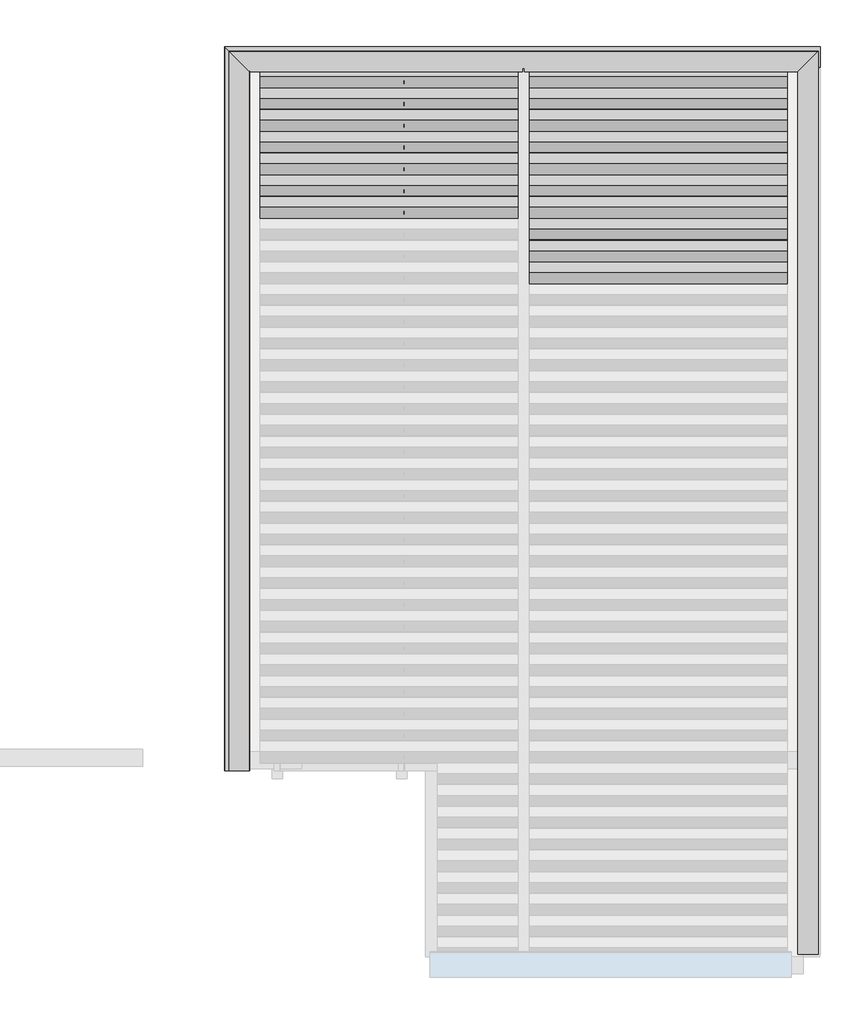
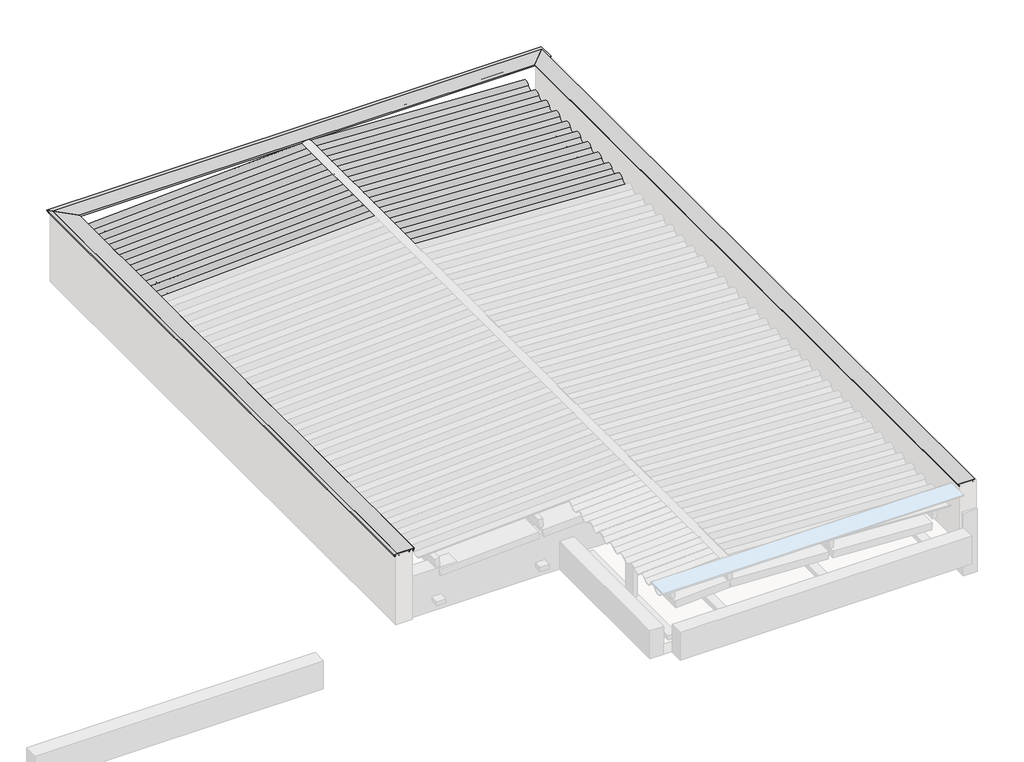
# One storey, part 4 of 4: 23 beams, 5 columns, 3 proxies.
"""IFC4 building model written with IfcOpenShell, lengths in millimetres."""

import ifcopenshell
import ifcopenshell.guid

model = None  # the IFC model being written
_history = None  # IfcOwnerHistory: only IFC2X3 demands one
_inside = {}  # id of a spatial element -> (the spatial element, [elements in it])
_under = {}  # id of a project, library or spatial element -> (it, [spatial elements below it])
_declared = {}  # id of a project -> (the project, [libraries it declares])
_typed = {}  # id of a type object -> (the type object, [elements of that type])
_made_of = {}  # id of a material, layer set ... -> (it, [elements and type objects made of it])


def new_model(schema):
    """Start an empty IFC model of exactly this schema.

    Asked for "IFC4X3", IfcOpenShell would pick the latest addendum, in which some entities
    have other attributes; the version numbers below select the first issue.
    IFC2X3 requires an IfcOwnerHistory on every rooted entity: one is made here for all.
    """
    global model, _history
    if schema == "IFC4X3":
        model = ifcopenshell.file(schema_version=(4, 3, 0, 0))
    else:
        model = ifcopenshell.file(schema=schema)
    _inside.clear()
    _under.clear()
    _declared.clear()
    _typed.clear()
    _made_of.clear()
    _history = None
    if model.schema == "IFC2X3":
        org = make("IfcOrganization", Name="unknown")
        user = make(
            "IfcPersonAndOrganization",
            ThePerson=make("IfcPerson", FamilyName="unknown"),
            TheOrganization=org,
        )
        app = make(
            "IfcApplication",
            ApplicationDeveloper=org,
            Version="unknown",
            ApplicationFullName="unknown",
            ApplicationIdentifier="unknown",
        )
        _history = make(
            "IfcOwnerHistory",
            OwningUser=user,
            OwningApplication=app,
            ChangeAction="ADDED",
            CreationDate=0,
        )
    return model


def make(cls, **values):
    """One entity of the class cls with the attributes given. An attribute that is None is left unset."""
    return model.create_entity(
        cls, **{name: value for name, value in values.items() if value is not None}
    )


def rooted(cls, **values):
    """An entity with a GlobalId (a new one), such as an element, a storey or a relation."""
    return make(cls, GlobalId=ifcopenshell.guid.new(), OwnerHistory=_history, **values)


def si_unit(unit_type, name, prefix=None):
    """IfcSIUnit, for example si_unit("LENGTHUNIT", "METRE", prefix="MILLI")."""
    return make("IfcSIUnit", UnitType=unit_type, Prefix=prefix, Name=name)


def assignment(units):
    """IfcUnitAssignment: the units of a project."""
    return None if units is None else make("IfcUnitAssignment", Units=units)


def point(xyz):
    """IfcCartesianPoint."""
    return None if xyz is None else make("IfcCartesianPoint", Coordinates=xyz)


def direction(xyz):
    """IfcDirection."""
    return None if xyz is None else make("IfcDirection", DirectionRatios=xyz)


def frame(location, z_axis=None, x_axis=None):
    """IfcAxis2Placement3D, a coordinate frame: its origin and axes. An axis left out is left unset."""
    return make(
        "IfcAxis2Placement3D",
        Location=point(location),
        Axis=direction(z_axis),
        RefDirection=direction(x_axis),
    )


def frame_2d(location, x_axis=None):
    """IfcAxis2Placement2D, a coordinate frame in the plane: its origin and x axis."""
    return make(
        "IfcAxis2Placement2D", Location=point(location), RefDirection=direction(x_axis)
    )


def origin():
    """The frame at (0, 0, 0) with its axes left unset."""
    return frame((0.0, 0.0, 0.0))


def place(relative_to, where):
    """IfcLocalPlacement: puts the frame where relative to a parent placement (None: the world)."""
    return make(
        "IfcLocalPlacement", PlacementRelTo=relative_to, RelativePlacement=where
    )


def context(
    kind, dimensions, precision=None, world=None, true_north=None, identifier=None
):
    """IfcGeometricRepresentationContext, for example the 3D "Model" context."""
    return make(
        "IfcGeometricRepresentationContext",
        ContextIdentifier=identifier,
        ContextType=kind,
        CoordinateSpaceDimension=dimensions,
        Precision=precision,
        WorldCoordinateSystem=world,
        TrueNorth=true_north,
    )


def project(units=None, contexts=None):
    """IfcProject with its units and contexts."""
    return rooted(
        "IfcProject",
        Name="project",
        RepresentationContexts=contexts,
        UnitsInContext=assignment(units),
    )


def spatial(cls, under=None, at=None, **own):
    """A site, building, storey or space (cls), placed at a placement, below another one or the project."""
    s = rooted(cls, ObjectPlacement=at, **own)
    if under is not None:
        _under.setdefault(under.id(), (under, []))[1].append(s)
    return s


def polyline(points):
    """IfcPolyline through the points."""
    return make("IfcPolyline", Points=[point(p) for p in points])


def circle_curve(where, radius):
    """IfcCircle in the frame where."""
    return make("IfcCircle", Position=where, Radius=radius)


def trimmed(basis, trim1, trim2, sense, master):
    """IfcTrimmedCurve: the piece of a basis curve between two trims."""
    return make(
        "IfcTrimmedCurve",
        BasisCurve=basis,
        Trim1=trim1,
        Trim2=trim2,
        SenseAgreement=sense,
        MasterRepresentation=master,
    )


def segment(curve, same_sense, transition):
    """IfcCompositeCurveSegment."""
    return make(
        "IfcCompositeCurveSegment",
        Transition=transition,
        SameSense=same_sense,
        ParentCurve=curve,
    )


def composite_curve(segments, self_intersect=None):
    """IfcCompositeCurve: segments joined end to end."""
    return make("IfcCompositeCurve", Segments=segments, SelfIntersect=self_intersect)


def outline(outer, holes=None, kind="AREA"):
    """IfcArbitraryClosedProfileDef: a profile drawn as a closed curve; with holes, ...WithVoids."""
    if holes is None:
        return make("IfcArbitraryClosedProfileDef", ProfileType=kind, OuterCurve=outer)
    return make(
        "IfcArbitraryProfileDefWithVoids",
        ProfileType=kind,
        OuterCurve=outer,
        InnerCurves=holes,
    )


def extrude(swept, where, along, depth):
    """IfcExtrudedAreaSolid: the profile swept, set in the frame where, extruded along a direction by depth."""
    return make(
        "IfcExtrudedAreaSolid",
        SweptArea=swept,
        Position=where,
        ExtrudedDirection=direction(along),
        Depth=depth,
    )


def faces_of(points, faces, orient=None, outer=None):
    """IfcFace entities. A face is a list of loops; a loop is a list of indices into points, from 0.

    orient and outer hold one flag for each loop. By default every Orientation is true, the
    first loop of a face is its IfcFaceOuterBound and the others are IfcFaceBound.
    """
    made = []
    for i, loops in enumerate(faces):
        bounds = []
        for j, loop in enumerate(loops):
            is_outer = j == 0 if outer is None else outer[i][j]
            bounds.append(
                make(
                    "IfcFaceOuterBound" if is_outer else "IfcFaceBound",
                    Bound=make("IfcPolyLoop", Polygon=[points[k] for k in loop]),
                    Orientation=True if orient is None else orient[i][j],
                )
            )
        made.append(make("IfcFace", Bounds=bounds))
    return made


def faceted_brep(points, faces, orient=None, outer=None, voids=None):
    """IfcFacetedBrep: a solid bounded by flat faces; with voids (closed shells), ...WithVoids."""
    shared = [point(p) for p in points]
    hull = make("IfcClosedShell", CfsFaces=faces_of(shared, faces, orient, outer))
    if voids is None:
        return make("IfcFacetedBrep", Outer=hull)
    return make(
        "IfcFacetedBrepWithVoids",
        Outer=hull,
        Voids=[
            make(cls, CfsFaces=faces_of(shared, fs, o, b)) for cls, fs, o, b in voids
        ],
    )


def shape(context_of_items, identifier, shape_type, items):
    """IfcShapeRepresentation: the items that make up one representation, for example the "Body"."""
    return make(
        "IfcShapeRepresentation",
        ContextOfItems=context_of_items,
        RepresentationIdentifier=identifier,
        RepresentationType=shape_type,
        Items=items,
    )


def source(mapping_origin, context_of_items, identifier, shape_type, items):
    """IfcRepresentationMap: a shape defined once, which mapped items show again and again."""
    return make(
        "IfcRepresentationMap",
        MappingOrigin=mapping_origin,
        MappedRepresentation=shape(context_of_items, identifier, shape_type, items),
    )


def transform(
    local_origin,
    x_axis=None,
    y_axis=None,
    z_axis=None,
    scale=None,
    scale2=None,
    scale3=None,
    uniform=True,
):
    """IfcCartesianTransformationOperator3D, or its non-uniform kind. x_axis, y_axis, z_axis: its Axis1, 2, 3."""
    if uniform:
        return make(
            "IfcCartesianTransformationOperator3D",
            Axis1=direction(x_axis),
            Axis2=direction(y_axis),
            LocalOrigin=point(local_origin),
            Scale=scale,
            Axis3=direction(z_axis),
        )
    return make(
        "IfcCartesianTransformationOperator3DnonUniform",
        Axis1=direction(x_axis),
        Axis2=direction(y_axis),
        LocalOrigin=point(local_origin),
        Scale=scale,
        Axis3=direction(z_axis),
        Scale2=scale2,
        Scale3=scale3,
    )


def mapped(mapping_source, mapping_target):
    """IfcMappedItem: shows the shape of a source again, moved by a transform."""
    return make(
        "IfcMappedItem", MappingSource=mapping_source, MappingTarget=mapping_target
    )


def made_of(thing, what):
    """Note that an element or type object is made of a material, layer set ...; save() writes the relation."""
    if what is not None:
        _made_of.setdefault(what.id(), (what, []))[1].append(thing)
    return thing


def element(
    cls,
    number,
    at=None,
    inside=None,
    cuts=None,
    type_object=None,
    material=None,
    context=None,
    identifier="Body",
    shape_type=None,
    held_by="IfcProductDefinitionShape",
    body=None,
    shapes=None,
    **own,
):
    """One element of the class cls, such as IfcWall. Its Tag is "e" and its number.

    at: its placement. inside: the storey or other place that contains it. cuts: it is an
    opening in that element (IfcRelVoidsElement). A single representation is given by context,
    identifier, shape_type and body (its items); several are given by shapes. held_by: the class
    of the entity that holds the representations. save() writes the other relations.
    """
    e = rooted(cls, Tag="e%d" % number, ObjectPlacement=at, **own)
    if body is not None:
        shapes = [shape(context, identifier, shape_type, body)]
    if shapes is not None:
        e.Representation = make(held_by, Representations=shapes)
    if inside is not None:
        _inside.setdefault(inside.id(), (inside, []))[1].append(e)
    if cuts is not None:
        rooted(
            "IfcRelVoidsElement", RelatingBuildingElement=cuts, RelatedOpeningElement=e
        )
    if type_object is not None:
        _typed.setdefault(type_object.id(), (type_object, []))[1].append(e)
    return made_of(e, material)


def aggregate(whole, parts):
    """IfcRelAggregates: a whole, such as a stair, and the parts it consists of."""
    return rooted("IfcRelAggregates", RelatingObject=whole, RelatedObjects=parts)


def save(model, path):
    """Write the relations noted so far, then the file.

    IfcRelAggregates (storeys below a building ...), IfcRelContainedInSpatialStructure (elements
    in a storey), IfcRelDefinesByType, IfcRelAssociatesMaterial and IfcRelDeclares: one each for
    every whole, place, type object, material and project.
    """
    for whole, parts in _under.values():
        aggregate(whole, parts)
    for where, things in _inside.values():
        rooted(
            "IfcRelContainedInSpatialStructure",
            RelatedElements=things,
            RelatingStructure=where,
        )
    for kind, things in _typed.values():
        rooted("IfcRelDefinesByType", RelatedObjects=things, RelatingType=kind)
    for what, things in _made_of.values():
        rooted("IfcRelAssociatesMaterial", RelatedObjects=things, RelatingMaterial=what)
    for by, libraries in _declared.values():
        rooted("IfcRelDeclares", RelatingContext=by, RelatedDefinitions=libraries)
    model.write(path)


def column_f3930958(model_context):
    return source(origin(), model_context, "Body", "SweptSolid", [
        extrude(outline(polyline([(30.0, 80.0), (30.0, -80.0), (-30.0, -80.0), (-30.0, 80.0), (30.0, 80.0)])), frame((0.0, 0.0, 4460.0), z_axis=(0.0, 0.0, 1.0), x_axis=(1.0, 0.0, 0.0)), (0.0, 0.0, 1.0), 522.9),
    ])


def column_4d3918cc(model_context):
    return source(origin(), model_context, "Body", "SweptSolid", [
        extrude(outline(polyline([(30.0, 80.0), (30.0, -80.0), (-30.0, -80.0), (-30.0, 80.0), (30.0, 80.0)])), frame((0.0, 0.0, 4460.0), z_axis=(0.0, 0.0, 1.0), x_axis=(1.0, 0.0, 0.0)), (0.0, 0.0, 1.0), 426.9),
    ])


def column_924cc83b(model_context):
    return source(origin(), model_context, "Body", "SweptSolid", [
        extrude(outline(polyline([(30.0, 80.0), (30.0, -80.0), (-30.0, -80.0), (-30.0, 80.0), (30.0, 80.0)])), frame((0.0, 0.0, 4460.0), z_axis=(0.0, 0.0, 1.0), x_axis=(1.0, 0.0, 0.0)), (0.0, 0.0, 1.0), 497.0),
    ])


model = new_model("IFC4")

# Units and contexts
model_context = context("Model", 3, world=origin())
ifc_project = project(units=[si_unit("LENGTHUNIT", "METRE", prefix="MILLI")], contexts=[model_context])

# Site, building, storey
site = spatial("IfcSite", under=ifc_project)
building = spatial("IfcBuilding", under=site)
storey = spatial("IfcBuildingStorey", under=building, Name="COB. SALA ESTAR", Elevation=4400.0)

# Beams
placement = place(None, origin())
element("IfcBeam", 1, ObjectType="Madeira de lei : Berço 6x12cm", at=placement, inside=storey, context=model_context, shape_type="SweptSolid", body=[
    extrude(outline(polyline([(-3400.781307, 5593.9300153), (-3280.781307, 5593.9300153), (-3280.781307, 3623.9300153), (-3400.781307, 3623.9300153), (-3400.781307, 5593.9300153)])), frame((0.0, 0.0, 4400.0), z_axis=(0.0, 0.0, 1.0), x_axis=(1.0, 0.0, 0.0)), (0.0, 0.0, 1.0), 60.0),
])
element("IfcBeam", 2, ObjectType="Madeira de lei : Berço 6x12cm", at=placement, inside=storey, context=model_context, shape_type="SweptSolid", body=[
    extrude(outline(polyline([(-2032.4438771, 5593.9300153), (-1912.4438771, 5593.9300153), (-1912.4438771, 3623.9300153), (-2032.4438771, 3623.9300153), (-2032.4438771, 5593.9300153)])), frame((0.0, 0.0, 4400.0), z_axis=(0.0, 0.0, 1.0), x_axis=(1.0, 0.0, 0.0)), (0.0, 0.0, 1.0), 60.0),
])
element("IfcBeam", 3, ObjectType="Madeira de lei : Berço 6x12cm", at=placement, inside=storey, context=model_context, shape_type="SweptSolid", body=[
    extrude(outline(polyline([(-634.1438771, 5593.9300153), (-514.1438771, 5593.9300153), (-514.1438771, 3623.9300153), (-634.1438771, 3623.9300153), (-634.1438771, 5593.9300153)])), frame((0.0, 0.0, 4400.0), z_axis=(0.0, 0.0, 1.0), x_axis=(1.0, 0.0, 0.0)), (0.0, 0.0, 1.0), 60.0),
])
element("IfcBeam", 4, ObjectType="Madeira de lei : Berço 6x12cm", at=placement, inside=storey, context=model_context, shape_type="SweptSolid", body=[
    extrude(outline(polyline([(-4769.1187368, 5593.9300153), (-4649.1187368, 5593.9300153), (-4649.1187368, 3623.9300153), (-4769.1187368, 3623.9300153), (-4769.1187368, 5593.9300153)])), frame((0.0, 0.0, 4400.0), z_axis=(0.0, 0.0, 1.0), x_axis=(1.0, 0.0, 0.0)), (0.0, 0.0, 1.0), 60.0),
])
element("IfcBeam", 5, ObjectType="Madeira de lei : Berço 6x12cm", at=placement, inside=storey, context=model_context, shape_type="SweptSolid", body=[
    extrude(outline(polyline([(-6167.4187368, 5593.9300153), (-6047.4187368, 5593.9300153), (-6047.4187368, 3623.9300153), (-6167.4187368, 3623.9300153), (-6167.4187368, 5593.9300153)])), frame((0.0, 0.0, 4400.0), z_axis=(0.0, 0.0, 1.0), x_axis=(1.0, 0.0, 0.0)), (0.0, 0.0, 1.0), 60.0),
])
element("IfcBeam", 6, ObjectType="TQS - Viga retangular : 19.0 x 60.0", at=placement, inside=storey, context=model_context, shape_type="SweptSolid", body=[
    extrude(outline(polyline([(-412.281307, 5774.4300153), (-412.281307, 5584.4300153), (-6230.281307, 5584.4300153), (-6230.281307, 5774.4300153), (-412.281307, 5774.4300153)])), frame((0.0, 0.0, 4250.0), z_axis=(0.0, 0.0, 1.0), x_axis=(1.0, 0.0, 0.0)), (0.0, 0.0, 1.0), 600.0),
])
element("IfcBeam", 7, ObjectType="Telha Ondulada : Fibrocimento", at=placement, inside=storey, context=model_context, shape_type="SweptSolid", body=[
    extrude(outline(composite_curve([segment(trimmed(circle_curve(frame_2d((-58.7002978, -53.2060538)), 66.7939461), [point((-29.3501488, 6.7939462))], [point((-29.3501488, -113.2060538))], False, "CARTESIAN"), True, "CONTINUOUS"), segment(polyline([(-29.3501488, -113.2060538), (-31.5472154, -108.7146288)]), True, "CONTINUOUS"), segment(trimmed(circle_curve(frame_2d((-58.7002978, -53.2060538)), 61.7939461), [point((-31.5472154, -108.7146288))], [point((-31.5472154, 2.3025211))], True, "CARTESIAN"), True, "CONTINUOUS"), segment(trimmed(circle_curve(frame_2d((0.0, 66.7939462)), 71.7939461), [point((-31.5472154, 2.3025211))], [point((-31.5472154, 131.2853712))], False, "CARTESIAN"), True, "CONTINUOUS"), segment(polyline([(-31.5472154, 131.2853712), (-29.3501488, 126.7939462)]), True, "CONTINUOUS"), segment(trimmed(circle_curve(frame_2d((0.0, 66.7939462)), 66.7939461), [point((-29.3501488, 126.7939462))], [point((-29.3501488, 6.7939462))], True, "CARTESIAN"), True, "CONTINUOUS")], self_intersect=False)), frame((-6303.6781287, 4045.326948, 5068.1236978), z_axis=(0.9987523388778448, 0.0, 0.04993761694389136), x_axis=(-0.04993761694389136, 0.0, 0.9987523388778448)), (0.0, 0.0, 1.0), 2962.0084336),
])
element("IfcBeam", 8, ObjectType="Telha Ondulada : Fibrocimento", at=placement, inside=storey, context=model_context, shape_type="SweptSolid", body=[
    extrude(outline(composite_curve([segment(trimmed(circle_curve(frame_2d((-58.7002978, -53.2060538)), 66.7939461), [point((-29.3501488, 6.7939462))], [point((-29.3501488, -113.2060538))], False, "CARTESIAN"), True, "CONTINUOUS"), segment(polyline([(-29.3501488, -113.2060538), (-31.5472154, -108.7146288)]), True, "CONTINUOUS"), segment(trimmed(circle_curve(frame_2d((-58.7002978, -53.2060538)), 61.7939461), [point((-31.5472154, -108.7146288))], [point((-31.5472154, 2.3025211))], True, "CARTESIAN"), True, "CONTINUOUS"), segment(trimmed(circle_curve(frame_2d((0.0, 66.7939462)), 71.7939461), [point((-31.5472154, 2.3025211))], [point((-31.5472154, 131.2853712))], False, "CARTESIAN"), True, "CONTINUOUS"), segment(polyline([(-31.5472154, 131.2853712), (-29.3501488, 126.7939462)]), True, "CONTINUOUS"), segment(trimmed(circle_curve(frame_2d((0.0, 66.7939462)), 66.7939461), [point((-29.3501488, 126.7939462))], [point((-29.3501488, 6.7939462))], True, "CARTESIAN"), True, "CONTINUOUS")], self_intersect=False)), frame((-6303.6781287, 4289.826948, 5068.1236978), z_axis=(0.9987523388778448, 0.0, 0.04993761694389134), x_axis=(-0.04993761694389134, 0.0, 0.9987523388778448)), (0.0, 0.0, 1.0), 2962.0084336),
])
element("IfcBeam", 9, ObjectType="Telha Ondulada : Fibrocimento", at=placement, inside=storey, context=model_context, shape_type="SweptSolid", body=[
    extrude(outline(composite_curve([segment(trimmed(circle_curve(frame_2d((-58.7002978, -53.2060538)), 66.7939461), [point((-29.3501488, 6.7939462))], [point((-29.3501488, -113.2060538))], False, "CARTESIAN"), True, "CONTINUOUS"), segment(polyline([(-29.3501488, -113.2060538), (-31.5472154, -108.7146288)]), True, "CONTINUOUS"), segment(trimmed(circle_curve(frame_2d((-58.7002978, -53.2060538)), 61.7939461), [point((-31.5472154, -108.7146288))], [point((-31.5472154, 2.3025211))], True, "CARTESIAN"), True, "CONTINUOUS"), segment(trimmed(circle_curve(frame_2d((0.0, 66.7939462)), 71.7939461), [point((-31.5472154, 2.3025211))], [point((-31.5472154, 131.2853712))], False, "CARTESIAN"), True, "CONTINUOUS"), segment(polyline([(-31.5472154, 131.2853712), (-29.3501488, 126.7939462)]), True, "CONTINUOUS"), segment(trimmed(circle_curve(frame_2d((0.0, 66.7939462)), 66.7939461), [point((-29.3501488, 126.7939462))], [point((-29.3501488, 6.7939462))], True, "CARTESIAN"), True, "CONTINUOUS")], self_intersect=False)), frame((-6303.6781287, 4534.326948, 5068.1236978), z_axis=(0.9987523388778448, 0.0, 0.04993761694389133), x_axis=(-0.04993761694389133, 0.0, 0.9987523388778448)), (0.0, 0.0, 1.0), 2962.0084336),
])
element("IfcBeam", 10, ObjectType="Telha Ondulada : Fibrocimento", at=placement, inside=storey, context=model_context, shape_type="SweptSolid", body=[
    extrude(outline(composite_curve([segment(trimmed(circle_curve(frame_2d((-58.7002978, -53.2060538)), 66.7939461), [point((-29.3501488, 6.7939462))], [point((-29.3501488, -113.2060538))], False, "CARTESIAN"), True, "CONTINUOUS"), segment(polyline([(-29.3501488, -113.2060538), (-31.5472154, -108.7146288)]), True, "CONTINUOUS"), segment(trimmed(circle_curve(frame_2d((-58.7002978, -53.2060538)), 61.7939461), [point((-31.5472154, -108.7146288))], [point((-31.5472154, 2.3025211))], True, "CARTESIAN"), True, "CONTINUOUS"), segment(trimmed(circle_curve(frame_2d((0.0, 66.7939462)), 71.7939461), [point((-31.5472154, 2.3025211))], [point((-31.5472154, 131.2853712))], False, "CARTESIAN"), True, "CONTINUOUS"), segment(polyline([(-31.5472154, 131.2853712), (-29.3501488, 126.7939462)]), True, "CONTINUOUS"), segment(trimmed(circle_curve(frame_2d((0.0, 66.7939462)), 66.7939461), [point((-29.3501488, 126.7939462))], [point((-29.3501488, 6.7939462))], True, "CARTESIAN"), True, "CONTINUOUS")], self_intersect=False)), frame((-6303.6781287, 4778.826948, 5068.1236978), z_axis=(0.9987523388778448, 0.0, 0.049937616943891344), x_axis=(-0.049937616943891344, 0.0, 0.9987523388778448)), (0.0, 0.0, 1.0), 2962.0084336),
])
element("IfcBeam", 11, ObjectType="Telha Ondulada : Fibrocimento", at=placement, inside=storey, context=model_context, shape_type="SweptSolid", body=[
    extrude(outline(composite_curve([segment(trimmed(circle_curve(frame_2d((-58.7002978, -53.2060538)), 66.7939461), [point((-29.3501488, 6.7939462))], [point((-29.3501488, -113.2060538))], False, "CARTESIAN"), True, "CONTINUOUS"), segment(polyline([(-29.3501488, -113.2060538), (-31.5472154, -108.7146288)]), True, "CONTINUOUS"), segment(trimmed(circle_curve(frame_2d((-58.7002978, -53.2060538)), 61.7939461), [point((-31.5472154, -108.7146288))], [point((-31.5472154, 2.3025211))], True, "CARTESIAN"), True, "CONTINUOUS"), segment(trimmed(circle_curve(frame_2d((0.0, 66.7939462)), 71.7939461), [point((-31.5472154, 2.3025211))], [point((-31.5472154, 131.2853712))], False, "CARTESIAN"), True, "CONTINUOUS"), segment(polyline([(-31.5472154, 131.2853712), (-29.3501488, 126.7939462)]), True, "CONTINUOUS"), segment(trimmed(circle_curve(frame_2d((0.0, 66.7939462)), 66.7939461), [point((-29.3501488, 126.7939462))], [point((-29.3501488, 6.7939462))], True, "CARTESIAN"), True, "CONTINUOUS")], self_intersect=False)), frame((-6303.6781287, 5023.326948, 5068.1236978), z_axis=(0.9987523388778448, 0.0, 0.04993761694389134), x_axis=(-0.04993761694389134, 0.0, 0.9987523388778448)), (0.0, 0.0, 1.0), 2962.0084336),
])
element("IfcBeam", 12, ObjectType="Telha Ondulada : Fibrocimento", at=placement, inside=storey, context=model_context, shape_type="SweptSolid", body=[
    extrude(outline(composite_curve([segment(trimmed(circle_curve(frame_2d((-58.7002978, -53.2060538)), 66.7939461), [point((-29.3501488, 6.7939462))], [point((-29.3501488, -113.2060538))], False, "CARTESIAN"), True, "CONTINUOUS"), segment(polyline([(-29.3501488, -113.2060538), (-31.5472154, -108.7146288)]), True, "CONTINUOUS"), segment(trimmed(circle_curve(frame_2d((-58.7002978, -53.2060538)), 61.7939461), [point((-31.5472154, -108.7146288))], [point((-31.5472154, 2.3025211))], True, "CARTESIAN"), True, "CONTINUOUS"), segment(trimmed(circle_curve(frame_2d((0.0, 66.7939462)), 71.7939461), [point((-31.5472154, 2.3025211))], [point((-31.5472154, 131.2853712))], False, "CARTESIAN"), True, "CONTINUOUS"), segment(polyline([(-31.5472154, 131.2853712), (-29.3501488, 126.7939462)]), True, "CONTINUOUS"), segment(trimmed(circle_curve(frame_2d((0.0, 66.7939462)), 66.7939461), [point((-29.3501488, 126.7939462))], [point((-29.3501488, 6.7939462))], True, "CARTESIAN"), True, "CONTINUOUS")], self_intersect=False)), frame((-6303.6781287, 5267.826948, 5068.1236978), z_axis=(0.9987523388778448, 0.0, 0.04993761694389136), x_axis=(-0.04993761694389136, 0.0, 0.9987523388778448)), (0.0, 0.0, 1.0), 2962.0084336),
])
element("IfcBeam", 13, ObjectType="Telha Ondulada : Fibrocimento", at=placement, inside=storey, context=model_context, shape_type="SweptSolid", body=[
    extrude(outline(composite_curve([segment(trimmed(circle_curve(frame_2d((-58.7002978, -53.2060538)), 66.7939461), [point((-29.3501488, 6.7939462))], [point((-29.3501488, -113.2060538))], False, "CARTESIAN"), True, "CONTINUOUS"), segment(polyline([(-29.3501488, -113.2060538), (-31.5472154, -108.7146288)]), True, "CONTINUOUS"), segment(trimmed(circle_curve(frame_2d((-58.7002978, -53.2060538)), 61.7939461), [point((-31.5472154, -108.7146288))], [point((-31.5472154, 2.3025211))], True, "CARTESIAN"), True, "CONTINUOUS"), segment(trimmed(circle_curve(frame_2d((0.0, 66.7939462)), 71.7939461), [point((-31.5472154, 2.3025211))], [point((-31.5472154, 131.2853712))], False, "CARTESIAN"), True, "CONTINUOUS"), segment(polyline([(-31.5472154, 131.2853712), (-29.3501488, 126.7939462)]), True, "CONTINUOUS"), segment(trimmed(circle_curve(frame_2d((0.0, 66.7939462)), 66.7939461), [point((-29.3501488, 126.7939462))], [point((-29.3501488, 6.7939462))], True, "CARTESIAN"), True, "CONTINUOUS")], self_intersect=False)), frame((-6303.6781287, 5512.326948, 5068.1236978), z_axis=(0.9987523388778448, 0.0, 0.04993761694389134), x_axis=(-0.04993761694389134, 0.0, 0.9987523388778448)), (0.0, 0.0, 1.0), 2962.0084336),
])
element("IfcBeam", 14, ObjectType="Telha Ondulada : Fibrocimento", at=placement, inside=storey, context=model_context, shape_type="SweptSolid", body=[
    extrude(outline(composite_curve([segment(trimmed(circle_curve(frame_2d((0.0, 66.7939462)), 66.7939461), [point((29.3501488, 6.7939462))], [point((29.3501488, 126.7939462))], True, "CARTESIAN"), True, "CONTINUOUS"), segment(polyline([(29.3501488, 126.7939462), (31.5472154, 131.2853712)]), True, "CONTINUOUS"), segment(trimmed(circle_curve(frame_2d((0.0, 66.7939462)), 71.7939461), [point((31.5472154, 131.2853712))], [point((31.5472154, 2.3025211))], False, "CARTESIAN"), True, "CONTINUOUS"), segment(trimmed(circle_curve(frame_2d((58.7002978, -53.2060538)), 61.7939461), [point((31.5472154, 2.3025211))], [point((31.5472154, -108.7146288))], True, "CARTESIAN"), True, "CONTINUOUS"), segment(polyline([(31.5472154, -108.7146288), (29.3501488, -113.2060538)]), True, "CONTINUOUS"), segment(trimmed(circle_curve(frame_2d((58.7002978, -53.2060538)), 66.7939461), [point((29.3501488, -113.2060538))], [point((29.3501488, 6.7939462))], False, "CARTESIAN"), True, "CONTINUOUS")], self_intersect=False)), frame((-377.8844852, 3311.826948, 5068.1236978), z_axis=(-0.9987523388778448, 0.0, 0.049937616943891455), x_axis=(-0.049937616943891455, 0.0, -0.9987523388778448)), (0.0, 0.0, 1.0), 2962.0084336),
])
element("IfcBeam", 15, ObjectType="Telha Ondulada : Fibrocimento", at=placement, inside=storey, context=model_context, shape_type="SweptSolid", body=[
    extrude(outline(composite_curve([segment(trimmed(circle_curve(frame_2d((0.0, 66.7939462)), 66.7939461), [point((29.3501488, 6.7939462))], [point((29.3501488, 126.7939462))], True, "CARTESIAN"), True, "CONTINUOUS"), segment(polyline([(29.3501488, 126.7939462), (31.5472154, 131.2853712)]), True, "CONTINUOUS"), segment(trimmed(circle_curve(frame_2d((0.0, 66.7939462)), 71.7939461), [point((31.5472154, 131.2853712))], [point((31.5472154, 2.3025211))], False, "CARTESIAN"), True, "CONTINUOUS"), segment(trimmed(circle_curve(frame_2d((58.7002978, -53.2060538)), 61.7939461), [point((31.5472154, 2.3025211))], [point((31.5472154, -108.7146288))], True, "CARTESIAN"), True, "CONTINUOUS"), segment(polyline([(31.5472154, -108.7146288), (29.3501488, -113.2060538)]), True, "CONTINUOUS"), segment(trimmed(circle_curve(frame_2d((58.7002978, -53.2060538)), 66.7939461), [point((29.3501488, -113.2060538))], [point((29.3501488, 6.7939462))], False, "CARTESIAN"), True, "CONTINUOUS")], self_intersect=False)), frame((-377.8844852, 3556.326948, 5068.1236978), z_axis=(-0.9987523388778448, 0.0, 0.049937616943891455), x_axis=(-0.049937616943891455, 0.0, -0.9987523388778448)), (0.0, 0.0, 1.0), 2962.0084336),
])
element("IfcBeam", 16, ObjectType="Telha Ondulada : Fibrocimento", at=placement, inside=storey, context=model_context, shape_type="SweptSolid", body=[
    extrude(outline(composite_curve([segment(trimmed(circle_curve(frame_2d((0.0, 66.7939462)), 66.7939461), [point((29.3501488, 6.7939462))], [point((29.3501488, 126.7939462))], True, "CARTESIAN"), True, "CONTINUOUS"), segment(polyline([(29.3501488, 126.7939462), (31.5472154, 131.2853712)]), True, "CONTINUOUS"), segment(trimmed(circle_curve(frame_2d((0.0, 66.7939462)), 71.7939461), [point((31.5472154, 131.2853712))], [point((31.5472154, 2.3025211))], False, "CARTESIAN"), True, "CONTINUOUS"), segment(trimmed(circle_curve(frame_2d((58.7002978, -53.2060538)), 61.7939461), [point((31.5472154, 2.3025211))], [point((31.5472154, -108.7146288))], True, "CARTESIAN"), True, "CONTINUOUS"), segment(polyline([(31.5472154, -108.7146288), (29.3501488, -113.2060538)]), True, "CONTINUOUS"), segment(trimmed(circle_curve(frame_2d((58.7002978, -53.2060538)), 66.7939461), [point((29.3501488, -113.2060538))], [point((29.3501488, 6.7939462))], False, "CARTESIAN"), True, "CONTINUOUS")], self_intersect=False)), frame((-377.8844852, 3800.826948, 5068.1236978), z_axis=(-0.9987523388778448, 0.0, 0.049937616943891455), x_axis=(-0.049937616943891455, 0.0, -0.9987523388778448)), (0.0, 0.0, 1.0), 2962.0084336),
])
element("IfcBeam", 17, ObjectType="Telha Ondulada : Fibrocimento", at=placement, inside=storey, context=model_context, shape_type="SweptSolid", body=[
    extrude(outline(composite_curve([segment(trimmed(circle_curve(frame_2d((0.0, 66.7939462)), 66.7939461), [point((29.3501488, 6.7939462))], [point((29.3501488, 126.7939462))], True, "CARTESIAN"), True, "CONTINUOUS"), segment(polyline([(29.3501488, 126.7939462), (31.5472154, 131.2853712)]), True, "CONTINUOUS"), segment(trimmed(circle_curve(frame_2d((0.0, 66.7939462)), 71.7939461), [point((31.5472154, 131.2853712))], [point((31.5472154, 2.3025211))], False, "CARTESIAN"), True, "CONTINUOUS"), segment(trimmed(circle_curve(frame_2d((58.7002978, -53.2060538)), 61.7939461), [point((31.5472154, 2.3025211))], [point((31.5472154, -108.7146288))], True, "CARTESIAN"), True, "CONTINUOUS"), segment(polyline([(31.5472154, -108.7146288), (29.3501488, -113.2060538)]), True, "CONTINUOUS"), segment(trimmed(circle_curve(frame_2d((58.7002978, -53.2060538)), 66.7939461), [point((29.3501488, -113.2060538))], [point((29.3501488, 6.7939462))], False, "CARTESIAN"), True, "CONTINUOUS")], self_intersect=False)), frame((-377.8844852, 4045.326948, 5068.1236978), z_axis=(-0.9987523388778448, 0.0, 0.049937616943891455), x_axis=(-0.049937616943891455, 0.0, -0.9987523388778448)), (0.0, 0.0, 1.0), 2962.0084336),
])
element("IfcBeam", 18, ObjectType="Telha Ondulada : Fibrocimento", at=placement, inside=storey, context=model_context, shape_type="SweptSolid", body=[
    extrude(outline(composite_curve([segment(trimmed(circle_curve(frame_2d((0.0, 66.7939462)), 66.7939461), [point((29.3501488, 6.7939462))], [point((29.3501488, 126.7939462))], True, "CARTESIAN"), True, "CONTINUOUS"), segment(polyline([(29.3501488, 126.7939462), (31.5472154, 131.2853712)]), True, "CONTINUOUS"), segment(trimmed(circle_curve(frame_2d((0.0, 66.7939462)), 71.7939461), [point((31.5472154, 131.2853712))], [point((31.5472154, 2.3025211))], False, "CARTESIAN"), True, "CONTINUOUS"), segment(trimmed(circle_curve(frame_2d((58.7002978, -53.2060538)), 61.7939461), [point((31.5472154, 2.3025211))], [point((31.5472154, -108.7146288))], True, "CARTESIAN"), True, "CONTINUOUS"), segment(polyline([(31.5472154, -108.7146288), (29.3501488, -113.2060538)]), True, "CONTINUOUS"), segment(trimmed(circle_curve(frame_2d((58.7002978, -53.2060538)), 66.7939461), [point((29.3501488, -113.2060538))], [point((29.3501488, 6.7939462))], False, "CARTESIAN"), True, "CONTINUOUS")], self_intersect=False)), frame((-377.8844852, 4289.826948, 5068.1236978), z_axis=(-0.9987523388778448, 0.0, 0.049937616943891455), x_axis=(-0.049937616943891455, 0.0, -0.9987523388778448)), (0.0, 0.0, 1.0), 2962.0084336),
])
element("IfcBeam", 19, ObjectType="Telha Ondulada : Fibrocimento", at=placement, inside=storey, context=model_context, shape_type="SweptSolid", body=[
    extrude(outline(composite_curve([segment(trimmed(circle_curve(frame_2d((0.0, 66.7939462)), 66.7939461), [point((29.3501488, 6.7939462))], [point((29.3501488, 126.7939462))], True, "CARTESIAN"), True, "CONTINUOUS"), segment(polyline([(29.3501488, 126.7939462), (31.5472154, 131.2853712)]), True, "CONTINUOUS"), segment(trimmed(circle_curve(frame_2d((0.0, 66.7939462)), 71.7939461), [point((31.5472154, 131.2853712))], [point((31.5472154, 2.3025211))], False, "CARTESIAN"), True, "CONTINUOUS"), segment(trimmed(circle_curve(frame_2d((58.7002978, -53.2060538)), 61.7939461), [point((31.5472154, 2.3025211))], [point((31.5472154, -108.7146288))], True, "CARTESIAN"), True, "CONTINUOUS"), segment(polyline([(31.5472154, -108.7146288), (29.3501488, -113.2060538)]), True, "CONTINUOUS"), segment(trimmed(circle_curve(frame_2d((58.7002978, -53.2060538)), 66.7939461), [point((29.3501488, -113.2060538))], [point((29.3501488, 6.7939462))], False, "CARTESIAN"), True, "CONTINUOUS")], self_intersect=False)), frame((-377.8844852, 4534.326948, 5068.1236978), z_axis=(-0.9987523388778448, 0.0, 0.049937616943891455), x_axis=(-0.049937616943891455, 0.0, -0.9987523388778448)), (0.0, 0.0, 1.0), 2962.0084336),
])
element("IfcBeam", 20, ObjectType="Telha Ondulada : Fibrocimento", at=placement, inside=storey, context=model_context, shape_type="SweptSolid", body=[
    extrude(outline(composite_curve([segment(trimmed(circle_curve(frame_2d((0.0, 66.7939462)), 66.7939461), [point((29.3501488, 6.7939462))], [point((29.3501488, 126.7939462))], True, "CARTESIAN"), True, "CONTINUOUS"), segment(polyline([(29.3501488, 126.7939462), (31.5472154, 131.2853712)]), True, "CONTINUOUS"), segment(trimmed(circle_curve(frame_2d((0.0, 66.7939462)), 71.7939461), [point((31.5472154, 131.2853712))], [point((31.5472154, 2.3025211))], False, "CARTESIAN"), True, "CONTINUOUS"), segment(trimmed(circle_curve(frame_2d((58.7002978, -53.2060538)), 61.7939461), [point((31.5472154, 2.3025211))], [point((31.5472154, -108.7146288))], True, "CARTESIAN"), True, "CONTINUOUS"), segment(polyline([(31.5472154, -108.7146288), (29.3501488, -113.2060538)]), True, "CONTINUOUS"), segment(trimmed(circle_curve(frame_2d((58.7002978, -53.2060538)), 66.7939461), [point((29.3501488, -113.2060538))], [point((29.3501488, 6.7939462))], False, "CARTESIAN"), True, "CONTINUOUS")], self_intersect=False)), frame((-377.8844852, 4778.826948, 5068.1236978), z_axis=(-0.9987523388778448, 0.0, 0.049937616943891455), x_axis=(-0.049937616943891455, 0.0, -0.9987523388778448)), (0.0, 0.0, 1.0), 2962.0084336),
])
element("IfcBeam", 21, ObjectType="Telha Ondulada : Fibrocimento", at=placement, inside=storey, context=model_context, shape_type="SweptSolid", body=[
    extrude(outline(composite_curve([segment(trimmed(circle_curve(frame_2d((0.0, 66.7939462)), 66.7939461), [point((29.3501488, 6.7939462))], [point((29.3501488, 126.7939462))], True, "CARTESIAN"), True, "CONTINUOUS"), segment(polyline([(29.3501488, 126.7939462), (31.5472154, 131.2853712)]), True, "CONTINUOUS"), segment(trimmed(circle_curve(frame_2d((0.0, 66.7939462)), 71.7939461), [point((31.5472154, 131.2853712))], [point((31.5472154, 2.3025211))], False, "CARTESIAN"), True, "CONTINUOUS"), segment(trimmed(circle_curve(frame_2d((58.7002978, -53.2060538)), 61.7939461), [point((31.5472154, 2.3025211))], [point((31.5472154, -108.7146288))], True, "CARTESIAN"), True, "CONTINUOUS"), segment(polyline([(31.5472154, -108.7146288), (29.3501488, -113.2060538)]), True, "CONTINUOUS"), segment(trimmed(circle_curve(frame_2d((58.7002978, -53.2060538)), 66.7939461), [point((29.3501488, -113.2060538))], [point((29.3501488, 6.7939462))], False, "CARTESIAN"), True, "CONTINUOUS")], self_intersect=False)), frame((-377.8844852, 5023.326948, 5068.1236978), z_axis=(-0.9987523388778448, 0.0, 0.049937616943891455), x_axis=(-0.049937616943891455, 0.0, -0.9987523388778448)), (0.0, 0.0, 1.0), 2962.0084336),
])
element("IfcBeam", 22, ObjectType="Telha Ondulada : Fibrocimento", at=placement, inside=storey, context=model_context, shape_type="SweptSolid", body=[
    extrude(outline(composite_curve([segment(trimmed(circle_curve(frame_2d((0.0, 66.7939462)), 66.7939461), [point((29.3501488, 6.7939462))], [point((29.3501488, 126.7939462))], True, "CARTESIAN"), True, "CONTINUOUS"), segment(polyline([(29.3501488, 126.7939462), (31.5472154, 131.2853712)]), True, "CONTINUOUS"), segment(trimmed(circle_curve(frame_2d((0.0, 66.7939462)), 71.7939461), [point((31.5472154, 131.2853712))], [point((31.5472154, 2.3025211))], False, "CARTESIAN"), True, "CONTINUOUS"), segment(trimmed(circle_curve(frame_2d((58.7002978, -53.2060538)), 61.7939461), [point((31.5472154, 2.3025211))], [point((31.5472154, -108.7146288))], True, "CARTESIAN"), True, "CONTINUOUS"), segment(polyline([(31.5472154, -108.7146288), (29.3501488, -113.2060538)]), True, "CONTINUOUS"), segment(trimmed(circle_curve(frame_2d((58.7002978, -53.2060538)), 66.7939461), [point((29.3501488, -113.2060538))], [point((29.3501488, 6.7939462))], False, "CARTESIAN"), True, "CONTINUOUS")], self_intersect=False)), frame((-377.8844852, 5267.826948, 5068.1236978), z_axis=(-0.9987523388778448, 0.0, 0.049937616943891455), x_axis=(-0.049937616943891455, 0.0, -0.9987523388778448)), (0.0, 0.0, 1.0), 2962.0084336),
])
element("IfcBeam", 23, ObjectType="Telha Ondulada : Fibrocimento", at=placement, inside=storey, context=model_context, shape_type="SweptSolid", body=[
    extrude(outline(composite_curve([segment(trimmed(circle_curve(frame_2d((0.0, 66.7939462)), 66.7939461), [point((29.3501488, 6.7939462))], [point((29.3501488, 126.7939462))], True, "CARTESIAN"), True, "CONTINUOUS"), segment(polyline([(29.3501488, 126.7939462), (31.5472154, 131.2853712)]), True, "CONTINUOUS"), segment(trimmed(circle_curve(frame_2d((0.0, 66.7939462)), 71.7939461), [point((31.5472154, 131.2853712))], [point((31.5472154, 2.3025211))], False, "CARTESIAN"), True, "CONTINUOUS"), segment(trimmed(circle_curve(frame_2d((58.7002978, -53.2060538)), 61.7939461), [point((31.5472154, 2.3025211))], [point((31.5472154, -108.7146288))], True, "CARTESIAN"), True, "CONTINUOUS"), segment(polyline([(31.5472154, -108.7146288), (29.3501488, -113.2060538)]), True, "CONTINUOUS"), segment(trimmed(circle_curve(frame_2d((58.7002978, -53.2060538)), 66.7939461), [point((29.3501488, -113.2060538))], [point((29.3501488, 6.7939462))], False, "CARTESIAN"), True, "CONTINUOUS")], self_intersect=False)), frame((-377.8844852, 5512.326948, 5068.1236978), z_axis=(-0.9987523388778448, 0.0, 0.049937616943891455), x_axis=(-0.049937616943891455, 0.0, -0.9987523388778448)), (0.0, 0.0, 1.0), 2962.0084336),
])

# Proxies
element("IfcBuildingElementProxy", 24, Name=".CC_RUFO_PINGADEIRA_22 cm", ObjectType=".CC_RUFO_PINGADEIRA_22 cm", at=placement, inside=storey, context=model_context, shape_type="Brep", body=[
    faceted_brep([(-243.5024445, -4345.5699847, 5226.6820963), (-236.4313766, -4345.5699847, 5233.7531641), (-236.4313766, -4345.5699847, 5236.5815912), (-243.0054581, -4345.5699847, 5230.0075098), (-258.952748, -4345.5699847, 5260.0), (-35.6098659, -4345.5699847, 5260.0), (-51.5571559, -4345.5699847, 5230.0075098), (-58.1312373, -4345.5699847, 5236.5815912), (-58.1312373, -4345.5699847, 5233.7531641), (-51.0601695, -4345.5699847, 5226.6820963), (-32.281307, -4345.5699847, 5262.0), (-262.281307, -4345.5699847, 5262.0), (-243.5024445, 5582.2088778, 5226.6820963), (-262.281307, 5563.4300153, 5262.0), (-32.281307, 5793.4300153, 5262.0), (-51.0601695, 5774.6511528, 5226.6820963), (-58.1312373, 5767.580085, 5233.7531641), (-58.1312373, 5767.580085, 5236.5815912), (-51.5571559, 5774.1541664, 5230.0075098), (-35.6098659, 5790.1014563, 5260.0), (-258.952748, 5566.7585743, 5260.0), (-243.0054581, 5582.7058642, 5230.0075098), (-236.4313766, 5589.2799456, 5236.5815912), (-236.4313766, 5589.2799456, 5233.7531641)], [[[0, 1, 2, 3, 4, 5, 6, 7, 8, 9, 10, 11]], [[12, 13, 14, 15, 16, 17, 18, 19, 20, 21, 22, 23]], [[1, 0, 12, 23]], [[2, 1, 23, 22]], [[3, 2, 22, 21]], [[4, 3, 21, 20]], [[5, 4, 20, 19]], [[6, 5, 19, 18]], [[7, 6, 18, 17]], [[8, 7, 17, 16]], [[9, 8, 16, 15]], [[10, 9, 15, 14]], [[11, 10, 14, 13]], [[0, 11, 13, 12]]]),
    faceted_brep([(-243.5024445, 5582.2088778, 5226.6820963), (-236.4313766, 5589.2799456, 5233.7531641), (-236.4313766, 5589.2799456, 5236.5815912), (-243.0054581, 5582.7058642, 5230.0075098), (-258.952748, 5566.7585743, 5260.0), (-35.6098659, 5790.1014563, 5260.0), (-51.5571559, 5774.1541664, 5230.0075098), (-58.1312373, 5767.580085, 5236.5815912), (-58.1312373, 5767.580085, 5233.7531641), (-51.0601695, 5774.6511528, 5226.6820963), (-32.281307, 5793.4300153, 5262.0), (-262.281307, 5563.4300153, 5262.0), (-6438.0601695, 5582.2088778, 5226.6820963), (-6419.281307, 5563.4300153, 5262.0), (-6649.281307, 5793.4300153, 5262.0), (-6630.5024445, 5774.6511528, 5226.6820963), (-6623.4313766, 5767.580085, 5233.7531641), (-6623.4313766, 5767.580085, 5236.5815912), (-6630.0054581, 5774.1541664, 5230.0075098), (-6645.952748, 5790.1014563, 5260.0), (-6422.6098659, 5566.7585743, 5260.0), (-6438.5571559, 5582.7058642, 5230.0075098), (-6445.1312373, 5589.2799456, 5236.5815912), (-6445.1312373, 5589.2799456, 5233.7531641)], [[[0, 1, 2, 3, 4, 5, 6, 7, 8, 9, 10, 11]], [[12, 13, 14, 15, 16, 17, 18, 19, 20, 21, 22, 23]], [[1, 0, 12, 23]], [[2, 1, 23, 22]], [[3, 2, 22, 21]], [[4, 3, 21, 20]], [[5, 4, 20, 19]], [[6, 5, 19, 18]], [[7, 6, 18, 17]], [[8, 7, 17, 16]], [[9, 8, 16, 15]], [[10, 9, 15, 14]], [[11, 10, 14, 13]], [[0, 11, 13, 12]]]),
    faceted_brep([(-6438.0601695, 5582.2088778, 5226.6820963), (-6445.1312373, 5589.2799456, 5233.7531641), (-6445.1312373, 5589.2799456, 5236.5815912), (-6438.5571559, 5582.7058642, 5230.0075098), (-6422.6098659, 5566.7585743, 5260.0), (-6645.952748, 5790.1014563, 5260.0), (-6630.0054581, 5774.1541664, 5230.0075098), (-6623.4313766, 5767.580085, 5236.5815912), (-6623.4313766, 5767.580085, 5233.7531641), (-6630.5024445, 5774.6511528, 5226.6820963), (-6649.281307, 5793.4300153, 5262.0), (-6419.281307, 5563.4300153, 5262.0), (-6438.0601695, -2284.5699847, 5226.6820963), (-6419.281307, -2284.5699847, 5262.0), (-6649.281307, -2284.5699847, 5262.0), (-6630.5024445, -2284.5699847, 5226.6820963), (-6623.4313766, -2284.5699847, 5233.7531641), (-6623.4313766, -2284.5699847, 5236.5815912), (-6630.0054581, -2284.5699847, 5230.0075098), (-6645.952748, -2284.5699847, 5260.0), (-6422.6098659, -2284.5699847, 5260.0), (-6438.5571559, -2284.5699847, 5230.0075098), (-6445.1312373, -2284.5699847, 5236.5815912), (-6445.1312373, -2284.5699847, 5233.7531641)], [[[0, 1, 2, 3, 4, 5, 6, 7, 8, 9, 10, 11]], [[12, 13, 14, 15, 16, 17, 18, 19, 20, 21, 22, 23]], [[1, 0, 12, 23]], [[2, 1, 23, 22]], [[3, 2, 22, 21]], [[4, 3, 21, 20]], [[5, 4, 20, 19]], [[6, 5, 19, 18]], [[7, 6, 18, 17]], [[8, 7, 17, 16]], [[9, 8, 16, 15]], [[10, 9, 15, 14]], [[11, 10, 14, 13]], [[0, 11, 13, 12]]]),
])
element("IfcBuildingElementProxy", 25, Name=".CC_RUFO_PINGADEIRA_22 cm", ObjectType=".CC_RUFO_PINGADEIRA_22 cm", at=placement, inside=storey, context=model_context, shape_type="Brep", body=[
    faceted_brep([(-243.5024445, -4345.5699847, 5226.6820963), (-236.4313766, -4345.5699847, 5233.7531641), (-236.4313766, -4345.5699847, 5236.5815912), (-243.0054581, -4345.5699847, 5230.0075098), (-258.952748, -4345.5699847, 5260.0), (-35.6098659, -4345.5699847, 5260.0), (-51.5571559, -4345.5699847, 5230.0075098), (-58.1312373, -4345.5699847, 5236.5815912), (-58.1312373, -4345.5699847, 5233.7531641), (-51.0601695, -4345.5699847, 5226.6820963), (-32.281307, -4345.5699847, 5262.0), (-262.281307, -4345.5699847, 5262.0), (-243.5024445, 5582.2088778, 5226.6820963), (-262.281307, 5563.4300153, 5262.0), (-32.281307, 5793.4300153, 5262.0), (-51.0601695, 5774.6511528, 5226.6820963), (-58.1312373, 5767.580085, 5233.7531641), (-58.1312373, 5767.580085, 5236.5815912), (-51.5571559, 5774.1541664, 5230.0075098), (-35.6098659, 5790.1014563, 5260.0), (-258.952748, 5566.7585743, 5260.0), (-243.0054581, 5582.7058642, 5230.0075098), (-236.4313766, 5589.2799456, 5236.5815912), (-236.4313766, 5589.2799456, 5233.7531641)], [[[0, 1, 2, 3, 4, 5, 6, 7, 8, 9, 10, 11]], [[12, 13, 14, 15, 16, 17, 18, 19, 20, 21, 22, 23]], [[1, 0, 12, 23]], [[2, 1, 23, 22]], [[3, 2, 22, 21]], [[4, 3, 21, 20]], [[5, 4, 20, 19]], [[6, 5, 19, 18]], [[7, 6, 18, 17]], [[8, 7, 17, 16]], [[9, 8, 16, 15]], [[10, 9, 15, 14]], [[11, 10, 14, 13]], [[0, 11, 13, 12]]]),
    faceted_brep([(-10.281307, 5826.6511528, 5226.6820963), (-10.281307, 5845.4300153, 5262.0), (-10.281307, 5615.4300153, 5262.0), (-10.281307, 5634.2088778, 5226.6820963), (-10.281307, 5641.2799456, 5233.7531641), (-10.281307, 5641.2799456, 5236.5815912), (-10.281307, 5634.7058642, 5230.0075098), (-10.281307, 5618.7585743, 5260.0), (-10.281307, 5842.1014563, 5260.0), (-10.281307, 5826.1541664, 5230.0075098), (-10.281307, 5819.580085, 5236.5815912), (-10.281307, 5819.580085, 5233.7531641), (-6682.5024445, 5826.6511528, 5226.6820963), (-6675.4313766, 5819.580085, 5233.7531641), (-6675.4313766, 5819.580085, 5236.5815912), (-6682.0054581, 5826.1541664, 5230.0075098), (-6697.952748, 5842.1014563, 5260.0), (-6645.952748, 5790.1014563, 5260.0), (-6474.6098659, 5618.7585743, 5260.0), (-6490.5571559, 5634.7058642, 5230.0075098), (-6497.1312373, 5641.2799456, 5236.5815912), (-6497.1312373, 5641.2799456, 5233.7531641), (-6490.0601695, 5634.2088778, 5226.6820963), (-6471.281307, 5615.4300153, 5262.0), (-6649.281307, 5793.4300153, 5262.0), (-6701.281307, 5845.4300153, 5262.0)], [[[0, 1, 2, 3, 4, 5, 6, 7, 8, 9, 10, 11]], [[12, 13, 14, 15, 16, 17, 18, 19, 20, 21, 22, 23, 24, 25]], [[1, 0, 12, 25]], [[2, 1, 25, 24, 23]], [[3, 2, 23, 22]], [[4, 3, 22, 21]], [[5, 4, 21, 20]], [[6, 5, 20, 19]], [[7, 6, 19, 18]], [[8, 7, 18, 17, 16]], [[9, 8, 16, 15]], [[10, 9, 15, 14]], [[11, 10, 14, 13]], [[0, 11, 13, 12]]]),
    faceted_brep([(-6682.5024445, 5826.6511528, 5226.6820963), (-6701.281307, 5845.4300153, 5262.0), (-6649.281307, 5793.4300153, 5262.0), (-6471.281307, 5615.4300153, 5262.0), (-6490.0601695, 5634.2088778, 5226.6820963), (-6497.1312373, 5641.2799456, 5233.7531641), (-6497.1312373, 5641.2799456, 5236.5815912), (-6490.5571559, 5634.7058642, 5230.0075098), (-6474.6098659, 5618.7585743, 5260.0), (-6645.952748, 5790.1014563, 5260.0), (-6697.952748, 5842.1014563, 5260.0), (-6682.0054581, 5826.1541664, 5230.0075098), (-6675.4313766, 5819.580085, 5236.5815912), (-6675.4313766, 5819.580085, 5233.7531641), (-6682.5024445, -2284.5699847, 5226.6820963), (-6675.4313766, -2284.5699847, 5233.7531641), (-6675.4313766, -2284.5699847, 5236.5815912), (-6682.0054581, -2284.5699847, 5230.0075098), (-6697.952748, -2284.5699847, 5260.0), (-6474.6098659, -2284.5699847, 5260.0), (-6490.5571559, -2284.5699847, 5230.0075098), (-6497.1312373, -2284.5699847, 5236.5815912), (-6497.1312373, -2284.5699847, 5233.7531641), (-6490.0601695, -2284.5699847, 5226.6820963), (-6471.281307, -2284.5699847, 5262.0), (-6701.281307, -2284.5699847, 5262.0)], [[[0, 1, 2, 3, 4, 5, 6, 7, 8, 9, 10, 11, 12, 13]], [[14, 15, 16, 17, 18, 19, 20, 21, 22, 23, 24, 25]], [[1, 0, 14, 25]], [[3, 2, 1, 25, 24]], [[4, 3, 24, 23]], [[5, 4, 23, 22]], [[6, 5, 22, 21]], [[7, 6, 21, 20]], [[8, 7, 20, 19]], [[10, 9, 8, 19, 18]], [[11, 10, 18, 17]], [[12, 11, 17, 16]], [[13, 12, 16, 15]], [[0, 13, 15, 14]]]),
])
element("IfcBuildingElementProxy", 26, Name=".CC_RUFO_PINGADEIRA_22 cm", ObjectType=".CC_RUFO_PINGADEIRA_22 cm", at=placement, inside=storey, context=model_context, shape_type="Brep", body=[
    faceted_brep([(-243.5024445, -4345.5699847, 5226.6820963), (-236.4313766, -4345.5699847, 5233.7531641), (-236.4313766, -4345.5699847, 5236.5815912), (-243.0054581, -4345.5699847, 5230.0075098), (-258.952748, -4345.5699847, 5260.0), (-35.6098659, -4345.5699847, 5260.0), (-51.5571559, -4345.5699847, 5230.0075098), (-58.1312373, -4345.5699847, 5236.5815912), (-58.1312373, -4345.5699847, 5233.7531641), (-51.0601695, -4345.5699847, 5226.6820963), (-32.281307, -4345.5699847, 5262.0), (-262.281307, -4345.5699847, 5262.0), (-243.5024445, 5582.2088778, 5226.6820963), (-262.281307, 5563.4300153, 5262.0), (-32.281307, 5793.4300153, 5262.0), (-51.0601695, 5774.6511528, 5226.6820963), (-58.1312373, 5767.580085, 5233.7531641), (-58.1312373, 5767.580085, 5236.5815912), (-51.5571559, 5774.1541664, 5230.0075098), (-35.6098659, 5790.1014563, 5260.0), (-258.952748, 5566.7585743, 5260.0), (-243.0054581, 5582.7058642, 5230.0075098), (-236.4313766, 5589.2799456, 5236.5815912), (-236.4313766, 5589.2799456, 5233.7531641)], [[[0, 1, 2, 3, 4, 5, 6, 7, 8, 9, 10, 11]], [[12, 13, 14, 15, 16, 17, 18, 19, 20, 21, 22, 23]], [[1, 0, 12, 23]], [[2, 1, 23, 22]], [[3, 2, 22, 21]], [[4, 3, 21, 20]], [[5, 4, 20, 19]], [[6, 5, 19, 18]], [[7, 6, 18, 17]], [[8, 7, 17, 16]], [[9, 8, 16, 15]], [[10, 9, 15, 14]], [[11, 10, 14, 13]], [[0, 11, 13, 12]]]),
    faceted_brep([(-243.5024445, 5582.2088778, 5226.6820963), (-236.4313766, 5589.2799456, 5233.7531641), (-236.4313766, 5589.2799456, 5236.5815912), (-243.0054581, 5582.7058642, 5230.0075098), (-258.952748, 5566.7585743, 5260.0), (-35.6098659, 5790.1014563, 5260.0), (-51.5571559, 5774.1541664, 5230.0075098), (-58.1312373, 5767.580085, 5236.5815912), (-58.1312373, 5767.580085, 5233.7531641), (-51.0601695, 5774.6511528, 5226.6820963), (-32.281307, 5793.4300153, 5262.0), (-262.281307, 5563.4300153, 5262.0), (-6438.0601695, 5582.2088778, 5226.6820963), (-6419.281307, 5563.4300153, 5262.0), (-6471.281307, 5615.4300153, 5262.0), (-6649.281307, 5793.4300153, 5262.0), (-6630.5024445, 5774.6511528, 5226.6820963), (-6623.4313766, 5767.580085, 5233.7531641), (-6623.4313766, 5767.580085, 5236.5815912), (-6630.0054581, 5774.1541664, 5230.0075098), (-6645.952748, 5790.1014563, 5260.0), (-6474.6098659, 5618.7585743, 5260.0), (-6422.6098659, 5566.7585743, 5260.0), (-6438.5571559, 5582.7058642, 5230.0075098), (-6445.1312373, 5589.2799456, 5236.5815912), (-6445.1312373, 5589.2799456, 5233.7531641)], [[[0, 1, 2, 3, 4, 5, 6, 7, 8, 9, 10, 11]], [[12, 13, 14, 15, 16, 17, 18, 19, 20, 21, 22, 23, 24, 25]], [[1, 0, 12, 25]], [[2, 1, 25, 24]], [[3, 2, 24, 23]], [[4, 3, 23, 22]], [[5, 4, 22, 21, 20]], [[6, 5, 20, 19]], [[7, 6, 19, 18]], [[8, 7, 18, 17]], [[9, 8, 17, 16]], [[10, 9, 16, 15]], [[11, 10, 15, 14, 13]], [[0, 11, 13, 12]]]),
    faceted_brep([(-6438.0601695, 5582.2088778, 5226.6820963), (-6445.1312373, 5589.2799456, 5233.7531641), (-6445.1312373, 5589.2799456, 5236.5815912), (-6438.5571559, 5582.7058642, 5230.0075098), (-6422.6098659, 5566.7585743, 5260.0), (-6474.6098659, 5618.7585743, 5260.0), (-6645.952748, 5790.1014563, 5260.0), (-6630.0054581, 5774.1541664, 5230.0075098), (-6623.4313766, 5767.580085, 5236.5815912), (-6623.4313766, 5767.580085, 5233.7531641), (-6630.5024445, 5774.6511528, 5226.6820963), (-6649.281307, 5793.4300153, 5262.0), (-6471.281307, 5615.4300153, 5262.0), (-6419.281307, 5563.4300153, 5262.0), (-6438.0601695, -2284.5699847, 5226.6820963), (-6419.281307, -2284.5699847, 5262.0), (-6649.281307, -2284.5699847, 5262.0), (-6630.5024445, -2284.5699847, 5226.6820963), (-6623.4313766, -2284.5699847, 5233.7531641), (-6623.4313766, -2284.5699847, 5236.5815912), (-6630.0054581, -2284.5699847, 5230.0075098), (-6645.952748, -2284.5699847, 5260.0), (-6422.6098659, -2284.5699847, 5260.0), (-6438.5571559, -2284.5699847, 5230.0075098), (-6445.1312373, -2284.5699847, 5236.5815912), (-6445.1312373, -2284.5699847, 5233.7531641)], [[[0, 1, 2, 3, 4, 5, 6, 7, 8, 9, 10, 11, 12, 13]], [[14, 15, 16, 17, 18, 19, 20, 21, 22, 23, 24, 25]], [[1, 0, 14, 25]], [[2, 1, 25, 24]], [[3, 2, 24, 23]], [[4, 3, 23, 22]], [[6, 5, 4, 22, 21]], [[7, 6, 21, 20]], [[8, 7, 20, 19]], [[9, 8, 19, 18]], [[10, 9, 18, 17]], [[11, 10, 17, 16]], [[13, 12, 11, 16, 15]], [[0, 13, 15, 14]]]),
])

# Columns
column_shape = column_f3930958(model_context)
element("IfcColumn", 27, ObjectType="Madeira de lei-Coluna : Pontalete 6X16cm", at=placement, inside=storey, context=model_context, shape_type="MappedRepresentation", body=[
    mapped(column_shape, transform((-3340.781307, 4623.9300153, 0.0), x_axis=(1.0, 0.0, 0.0), y_axis=(0.0, 1.0, 0.0), z_axis=(0.0, 0.0, 1.0))),
])
column_2_shape = column_4d3918cc(model_context)
element("IfcColumn", 28, ObjectType="Madeira de lei-Coluna : Pontalete 6X16cm", at=placement, inside=storey, context=model_context, shape_type="MappedRepresentation", body=[
    mapped(column_2_shape, transform((-574.1438771, 4623.9300153, 0.0), x_axis=(1.0, 0.0, 0.0), y_axis=(0.0, 1.0, 0.0), z_axis=(0.0, 0.0, 1.0))),
])
element("IfcColumn", 29, ObjectType="Madeira de lei-Coluna : Pontalete 6X16cm", at=placement, inside=storey, context=model_context, shape_type="MappedRepresentation", body=[
    mapped(column_2_shape, transform((-6107.4187368, 4623.9300153, 0.0), x_axis=(1.0, 0.0, 0.0), y_axis=(0.0, 1.0, 0.0), z_axis=(0.0, 0.0, 1.0))),
])
column_3_shape = column_924cc83b(model_context)
element("IfcColumn", 30, ObjectType="Madeira de lei-Coluna : Pontalete 6X16cm", at=placement, inside=storey, context=model_context, shape_type="MappedRepresentation", body=[
    mapped(column_3_shape, transform((-1972.4438771, 4623.9300153, 0.0), x_axis=(1.0, 0.0, 0.0), y_axis=(0.0, 1.0, 0.0), z_axis=(0.0, 0.0, 1.0))),
])
element("IfcColumn", 31, ObjectType="Madeira de lei-Coluna : Pontalete 6X16cm", at=placement, inside=storey, context=model_context, shape_type="MappedRepresentation", body=[
    mapped(column_3_shape, transform((-4709.1187368, 4623.9300153, 0.0), x_axis=(1.0, 0.0, 0.0), y_axis=(0.0, 1.0, 0.0), z_axis=(0.0, 0.0, 1.0))),
])

save(model, "model.ifc")

# Revit data of these elements
# Type "Madeira de lei : Berço 6x12cm"
#   A = 0.02 m²
#   Length [instance default] = 1.524 m
#   b = 0.06 m
#   d = 0.12 m
#   Structural Material [instance default] = none
#   Assembly Code = ""
# Type "TQS - Viga retangular : 19.0 x 60.0"
#   Length [instance default] = 1.524 m
#   b = 0.19 m
#   h = 0.60 m
#   Structural Material [instance default] = none
#   Assembly Code = ""
# Type "Telha Ondulada : Fibrocimento"
#   Description = "TELHA ONDULADA FIBROCIMENTO"
#   Cost = 5
#   Length [instance default] = 1.524 m
#   b = 0.07 m
#   h = 0.16 m
#   Structural Material = .TELHA DE FIBROCIMENTO
#   Assembly Code = ""
# Type ".CC_RUFO_PINGADEIRA_22 cm"
#   Description = "RUFO METÁLICO"
# Type "Madeira de lei-Coluna : Pontalete 6X16cm"
#   A = 0.01952 m²
#   b = 0.06 m
#   d = 0.16 m
#   Structural Material [instance default] = none
#   Assembly Code = ""
# Elements 1, 2, 3, 4, 5 (IfcBeam, "Madeira de lei : Berço 6x12cm")
#   Comments = ""
#   Structural Material = .MADEIRAMENTO
#   Phase Created = CC_PE
#   Materials on its faces: ".MADEIRAMENTO"
# Element 6 (IfcBeam, "TQS - Viga retangular : 19.0 x 60.0")
#   Uso = "ESTRUTURA"
#   Titulo = "V301"
#   Chave = "-296"
#   Tipo Elemento = "Viga"
#   SHA1 = "757894CEA72A4CB6221DF2E576041B09F085C368"
#   Revisão = ""
#   Tipo de carga = ""
#   Divisor de flexao = ""
#   Secao = ""
#   Configuracao = ""
#   Angulo (graus) = ""
#   Detalhamento = ""
#   Casos de vento manual = ""
#   Tipo = ""
#   Alcas = ""
#   Furos = ""
#   Pino = ""
#   Distribuicao = ""
#   Solidarizado = ""
#   Solidarizar na montagem = ""
#   Unir com o próximo = ""
#   Grupo pre moldado = ""
#   Verificado = ""
#   Concreto C = ""
#   Taxa de armadura (kgf/m³) = 0
#   Carga (tf/m²) = 0
#   Carga (tf/m) = 0
#   Carga (tf) = 0
#   Altura = 0.60 m
#   Rebaixo = -0.45 m
#   Largura = 0.19 m
#   Distancia a face = 0.00 m
#   Distancia ao eixo = 0.00 m
#   Altura gerber esquerda = 0.00 m
#   Largura gerber esquerda = 0.00 m
#   Altura gerber direita = 0.00 m
#   Largura gerber direita = 0.00 m
#   Resultado de Ensaios fck (MPa) = 0
#   Unique TQS ID = -296
#   Principal = yes
#   Structural Material = none
#   Phase Created = CC_PE
# Elements 7, 8, 9, 10, 11, 12, 13, 14, 15, 16, 17, 18, 19, 20, 21, 22, 23 (IfcBeam, "Telha Ondulada : Fibrocimento")
#   Phase Created = CC_PE
#   Materials on its faces: ".TELHA DE FIBROCIMENTO"
# Elements 24, 26 (IfcBuildingElementProxy, ".CC_RUFO_PINGADEIRA_22 cm")
#   Uso = "RUFOS COB. SALA ESTAR/JANTAR"
#   Phase Created = CC_PE
